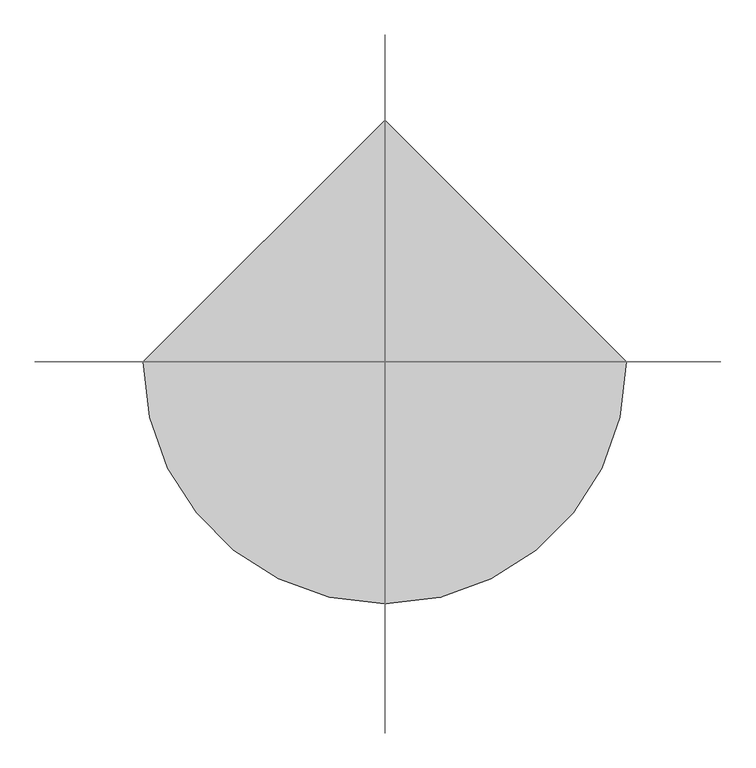
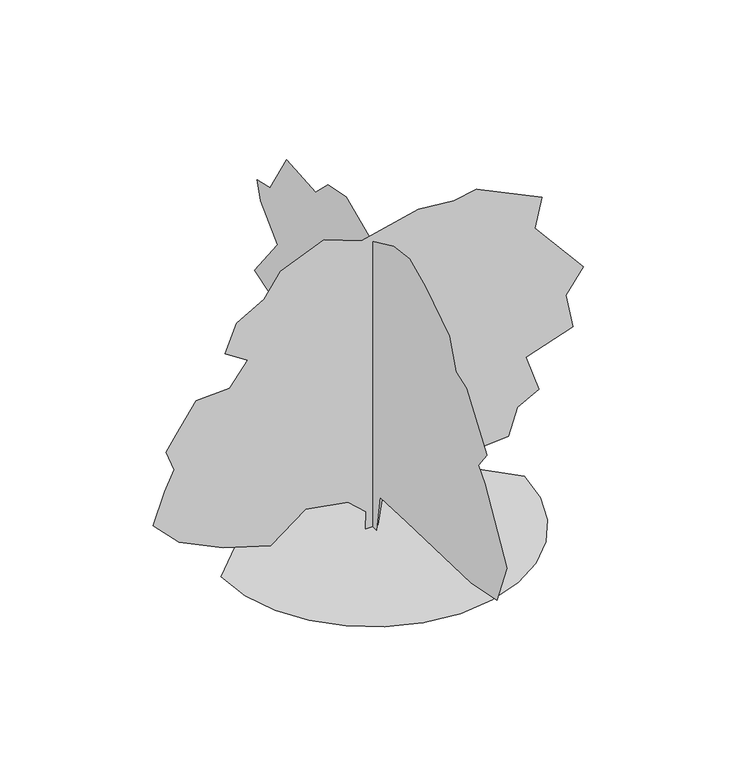
"""IFC4 building model written with IfcOpenShell, lengths in millimetres: proxy geometry, hibiscus syriacus 26076 : hibiscus syriacus 26076."""

from ifc_helpers import new_model, si_unit, origin, place, context, project, spatial, triangles, source, transform, mapped, element, save


def entourage_edde2c96(model_context):
    return source(origin(), model_context, "Body", "Tessellation", [
        triangles([(-718.2296339, 0.0, 5.8e-05), (-699.2430748, -164.5709867, 5.8e-05), (-645.166361, -315.7023142, 5.8e-05), (-560.3301876, -449.0652858, 5.8e-05), (-449.0652858, -560.3301876, 5.8e-05), (-315.7023142, -645.166361, 5.8e-05), (-164.5707324, -699.2430748, 5.8e-05), (3.14e-05, -718.2296339, 5.8e-05), (164.5709867, -699.2430748, 5.8e-05), (315.7023142, -645.166361, 5.8e-05), (449.0652858, -560.3301876, 5.8e-05), (560.3301876, -449.0652858, 5.8e-05), (645.166361, -315.7023142, 5.8e-05), (699.2430748, -164.5707324, 5.8e-05), (718.2296339, 6.28e-05, 5.8e-05), (-9.42e-05, 718.2296339, 5.8e-05), (-34.4417068, 8.54e-05, 0.0004029), (-31.4201161, 7.54e-05, 85.3357887), (-116.0190539, 6.6e-05, 163.8917949), (-318.4505839, 6.17e-05, 200.1483391), (-484.6279043, 7.68e-05, 73.2501891), (-708.2093153, 6.85e-05, 142.7419322), (-916.6853256, 5.67e-05, 242.4475559), (-1040.5638834, 4.15e-05, 369.3446795), (-986.1773048, 2.35e-05, 520.4140194), (-940.856016, 1.24e-05, 614.076689), (-980.1346504, 1e-07, 716.8046482), (-931.7932697, -8.2e-06, 786.2967001), (-838.1305275, -2.47e-05, 925.2806585), (-677.9959705, -2.55e-05, 931.323313), (-593.398518, -3.84e-05, 1040.0939993), (-699.1465691, -4.67e-05, 1109.5859785), (-644.762534, -6.29e-05, 1245.5473743), (-514.8412491, -7.16e-05, 1318.0593727), (-436.2865236, -8.53e-05, 1432.8727135), (-230.8316043, -9.53e-05, 1517.4726368), (-52.5699789, -8.74e-05, 1451.0008221), (216.3332524, -9.5e-05, 1514.4501469), (385.5321362, -9.28e-05, 1496.3220383), (491.2801509, -9.53e-05, 1517.4726368), (802.4816133, -7.77e-05, 1369.4233887), (769.2456333, -6.04e-05, 1224.3967758), (998.8722422, -2.8e-05, 952.4739841), (914.2723188, -1.43e-05, 837.6606434), (947.5082262, 5.9e-06, 668.4632675), (726.946907, 1.49e-05, 592.9286339), (787.37614, 3.65e-05, 411.6459128), (684.6481808, 4.3e-05, 357.2593343), (642.3495272, 5.85e-05, 227.340611), (237.483106, 6.21e-05, 197.1267394), (140.7988277, 7.07e-05, 124.6136692), (53.1785627, 6.42e-05, 178.9984673), (25.9860297, 8.59e-05, 0.0), (-0.0007807, 31.0927106, 0.000457), (-0.0007807, 31.0927106, 100.9481805), (-0.0007869, 87.072138, 68.5389896), (-0.0007995, 193.1381747, 80.3241033), (-0.0008058, 269.7409118, 130.4109715), (-0.0008121, 346.3449205, 98.0017761), (-0.0008373, 520.1752622, 192.282958), (-0.0008373, 470.0888935, 354.3281542), (-0.0008562, 649.8120077, 383.7922351), (-0.0008688, 764.7167673, 489.857745), (-0.0008688, 747.0383406, 566.4617901), (-0.0008877, 891.4071447, 584.1376734), (-0.0008814, 850.1600258, 657.7952414), (-0.0009003, 970.9575943, 696.098572), (-0.0008877, 782.3951941, 937.693709), (-0.0009066, 920.8711893, 1073.2207563), (-0.0009066, 950.3327631, 1161.6103466), (-0.0009003, 841.3208124, 1188.1254433), (-0.000894, 705.7912216, 1409.0982925), (-0.0008688, 470.0888935, 1388.4733887), (-0.0008562, 366.9697881, 1488.6486694), (-0.0008436, 219.6545613, 1518.1102432), (-0.0008184, 4.575997, 1426.7767193), (-0.0007995, -172.2011714, 1509.2709572), (-0.0007869, -301.8364273, 1524.0030521), (-0.0007744, -431.473191, 1462.131102), (-0.0007492, -628.8747683, 1335.4407246), (-0.0007366, -684.8539822, 1191.0718477), (-0.0007303, -770.297168, 1161.6103466), (-0.0007051, -938.2346643, 925.9080185), (-0.0007114, -867.5235008, 834.5720238), (-0.0007051, -920.5562376, 772.700001), (-0.0006736, -1103.2258289, 460.3937004), (-0.0006736, -1020.7315184, 251.2085401), (-0.0006988, -811.5442869, 209.9606217), (-0.0007555, -275.3213124, 192.282958), (-0.0007744, -60.2420624, 183.443999), (-0.0007744, -30.7792736, 0.0004496)], [[15, 16, 1], [14, 15, 1], [14, 1, 2], [13, 14, 2], [13, 2, 3], [13, 3, 4], [12, 13, 4], [11, 12, 4], [11, 4, 5], [11, 5, 6], [11, 6, 7], [11, 7, 8], [11, 8, 9], [11, 9, 10], [53, 17, 18], [52, 53, 18], [52, 18, 19], [44, 45, 46], [46, 47, 48], [31, 32, 33], [40, 41, 42], [42, 43, 44], [31, 33, 34], [50, 51, 52], [48, 49, 50], [23, 24, 25], [46, 48, 50], [42, 44, 46], [39, 40, 42], [39, 42, 46], [39, 46, 50], [38, 39, 50], [37, 38, 50], [37, 50, 52], [37, 52, 19], [37, 19, 20], [36, 37, 20], [35, 36, 20], [34, 35, 20], [31, 34, 20], [30, 31, 20], [30, 20, 21], [30, 21, 22], [30, 22, 23], [30, 23, 25], [30, 25, 26], [29, 30, 26], [28, 29, 26], [28, 26, 27], [64, 65, 66], [66, 67, 68], [69, 70, 71], [91, 54, 55], [90, 91, 55], [68, 69, 71], [59, 60, 61], [58, 59, 61], [82, 83, 84], [71, 72, 73], [68, 71, 73], [64, 66, 68], [62, 63, 64], [86, 87, 88], [85, 86, 88], [85, 88, 89], [84, 85, 89], [82, 84, 89], [81, 82, 89], [81, 89, 90], [80, 81, 90], [79, 80, 90], [78, 79, 90], [77, 78, 90], [76, 77, 90], [75, 76, 90], [74, 75, 90], [73, 74, 90], [68, 73, 90], [64, 68, 90], [64, 90, 55], [64, 55, 56], [61, 62, 64], [61, 64, 56], [58, 61, 56], [58, 56, 57]], closed=False),
    ])


if __name__ == "__main__":
    model = new_model("IFC4")
    model_context = context("Model", 3, world=origin())
    ifc_project = project(units=[si_unit("LENGTHUNIT", "METRE", prefix="MILLI")], contexts=[model_context])
    site = spatial("IfcSite", under=ifc_project)
    building = spatial("IfcBuilding", under=site)
    placement = place(None, origin())
    entourage_shape = entourage_edde2c96(model_context)
    element("IfcBuildingElementProxy", 1, Name="hibiscus syriacus 26076 : hibiscus syriacus 26076", ObjectType="hibiscus syriacus 26076 : hibiscus syriacus 26076", at=placement, inside=building, context=model_context, shape_type="MappedRepresentation", body=[
        mapped(entourage_shape, transform((0.0, 0.0, 0.0), x_axis=(1.0, 0.0, 0.0), y_axis=(0.0, 1.0, 0.0), z_axis=(0.0, 0.0, 1.0))),
    ])
    save(model, "model.ifc")

# Revit data of these elements
# Type "hibiscus syriacus 26076 : hibiscus syriacus 26076"
#   built-in parameter 1005195 = "RPC-16-FVPE-AH00-2TUK-G000-ST1L-LVER-AU"
#   Height = 0
